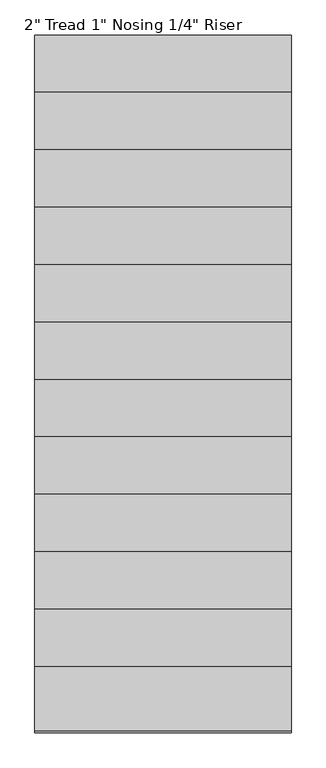
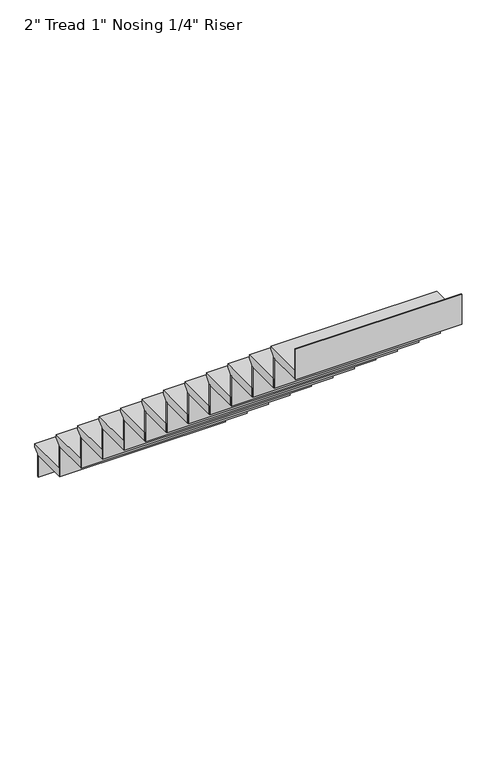
"""IFC4 building model written with IfcOpenShell, lengths in millimetres: stair flight geometry."""

from ifc_helpers import new_model, si_unit, frame, origin, place, context, project, spatial, polyline, outline, extrude, source, transform, mapped, element, save


def stair_flight_7df519db(model_context):
    return source(origin(), model_context, "Body", "SweptSolid", [
        extrude(outline(polyline([(-5623.7944564, -2092.5692308), (-5395.1944564, -2092.5692308), (-5395.1944564, -2111.6192308), (-5420.5944564, -2137.0192308), (-5420.5944564, -2143.3692308), (-5623.7944564, -2143.3692308), (-5623.7944564, -2092.5692308)])), frame((-2404.0095256, 0.0, 0.0), z_axis=(1.0, 0.0, 0.0), x_axis=(0.0, 1.0, 0.0)), (0.0, 0.0, 1.0), 908.05),
        extrude(outline(polyline([(-2404.0095256, -5426.9444564), (-2404.0095256, -5420.5944564), (-1495.9595256, -5420.5944564), (-1495.9595256, -5426.9444564), (-2404.0095256, -5426.9444564)])), frame((0.0, 0.0, -2266.95), z_axis=(0.0, 0.0, 1.0), x_axis=(1.0, 0.0, 0.0)), (0.0, 0.0, 1.0), 123.5807692),
        extrude(outline(polyline([(-2404.0095256, -5630.1444564), (-2404.0095256, -5623.7944564), (-1495.9595256, -5623.7944564), (-1495.9595256, -5630.1444564), (-2404.0095256, -5630.1444564)])), frame((0.0, 0.0, -2143.3692308), z_axis=(0.0, 0.0, 1.0), x_axis=(1.0, 0.0, 0.0)), (0.0, 0.0, 1.0), 174.3807692),
        extrude(outline(polyline([(-5826.9944564, -1918.1884615), (-5598.3944564, -1918.1884615), (-5598.3944564, -1937.2384615), (-5623.7944564, -1962.6384615), (-5623.7944564, -1968.9884615), (-5826.9944564, -1968.9884615), (-5826.9944564, -1918.1884615)])), frame((-2404.0095256, 0.0, 0.0), z_axis=(1.0, 0.0, 0.0), x_axis=(0.0, 1.0, 0.0)), (0.0, 0.0, 1.0), 908.05),
        extrude(outline(polyline([(-2404.0095256, -5833.3444564), (-2404.0095256, -5826.9944564), (-1495.9595256, -5826.9944564), (-1495.9595256, -5833.3444564), (-2404.0095256, -5833.3444564)])), frame((0.0, 0.0, -1968.9884615), z_axis=(0.0, 0.0, 1.0), x_axis=(1.0, 0.0, 0.0)), (0.0, 0.0, 1.0), 174.3807692),
        extrude(outline(polyline([(-6030.1944564, -1743.8076923), (-5801.5944564, -1743.8076923), (-5801.5944564, -1762.8576923), (-5826.9944564, -1788.2576923), (-5826.9944564, -1794.6076923), (-6030.1944564, -1794.6076923), (-6030.1944564, -1743.8076923)])), frame((-2404.0095256, 0.0, 0.0), z_axis=(1.0, 0.0, 0.0), x_axis=(0.0, 1.0, 0.0)), (0.0, 0.0, 1.0), 908.05),
        extrude(outline(polyline([(-2404.0095256, -6036.5444564), (-2404.0095256, -6030.1944564), (-1495.9595256, -6030.1944564), (-1495.9595256, -6036.5444564), (-2404.0095256, -6036.5444564)])), frame((0.0, 0.0, -1794.6076923), z_axis=(0.0, 0.0, 1.0), x_axis=(1.0, 0.0, 0.0)), (0.0, 0.0, 1.0), 174.3807692),
        extrude(outline(polyline([(-6233.3944564, -1569.4269231), (-6004.7944564, -1569.4269231), (-6004.7944564, -1588.4769231), (-6030.1944564, -1613.8769231), (-6030.1944564, -1620.2269231), (-6233.3944564, -1620.2269231), (-6233.3944564, -1569.4269231)])), frame((-2404.0095256, 0.0, 0.0), z_axis=(1.0, 0.0, 0.0), x_axis=(0.0, 1.0, 0.0)), (0.0, 0.0, 1.0), 908.05),
        extrude(outline(polyline([(-2404.0095256, -6239.7444564), (-2404.0095256, -6233.3944564), (-1495.9595256, -6233.3944564), (-1495.9595256, -6239.7444564), (-2404.0095256, -6239.7444564)])), frame((0.0, 0.0, -1620.2269231), z_axis=(0.0, 0.0, 1.0), x_axis=(1.0, 0.0, 0.0)), (0.0, 0.0, 1.0), 174.3807692),
        extrude(outline(polyline([(-6436.5944564, -1395.0461538), (-6207.9944564, -1395.0461538), (-6207.9944564, -1414.0961538), (-6233.3944564, -1439.4961538), (-6233.3944564, -1445.8461538), (-6436.5944564, -1445.8461538), (-6436.5944564, -1395.0461538)])), frame((-2404.0095256, 0.0, 0.0), z_axis=(1.0, 0.0, 0.0), x_axis=(0.0, 1.0, 0.0)), (0.0, 0.0, 1.0), 908.05),
        extrude(outline(polyline([(-2404.0095256, -6442.9444564), (-2404.0095256, -6436.5944564), (-1495.9595256, -6436.5944564), (-1495.9595256, -6442.9444564), (-2404.0095256, -6442.9444564)])), frame((0.0, 0.0, -1445.8461538), z_axis=(0.0, 0.0, 1.0), x_axis=(1.0, 0.0, 0.0)), (0.0, 0.0, 1.0), 174.3807692),
        extrude(outline(polyline([(-6639.7944564, -1220.6653846), (-6411.1944564, -1220.6653846), (-6411.1944564, -1239.7153846), (-6436.5944564, -1265.1153846), (-6436.5944564, -1271.4653846), (-6639.7944564, -1271.4653846), (-6639.7944564, -1220.6653846)])), frame((-2404.0095256, 0.0, 0.0), z_axis=(1.0, 0.0, 0.0), x_axis=(0.0, 1.0, 0.0)), (0.0, 0.0, 1.0), 908.05),
        extrude(outline(polyline([(-2404.0095256, -6646.1444564), (-2404.0095256, -6639.7944564), (-1495.9595256, -6639.7944564), (-1495.9595256, -6646.1444564), (-2404.0095256, -6646.1444564)])), frame((0.0, 0.0, -1271.4653846), z_axis=(0.0, 0.0, 1.0), x_axis=(1.0, 0.0, 0.0)), (0.0, 0.0, 1.0), 174.3807692),
        extrude(outline(polyline([(-6842.9944564, -1046.2846154), (-6614.3944564, -1046.2846154), (-6614.3944564, -1065.3346154), (-6639.7944564, -1090.7346154), (-6639.7944564, -1097.0846154), (-6842.9944564, -1097.0846154), (-6842.9944564, -1046.2846154)])), frame((-2404.0095256, 0.0, 0.0), z_axis=(1.0, 0.0, 0.0), x_axis=(0.0, 1.0, 0.0)), (0.0, 0.0, 1.0), 908.05),
        extrude(outline(polyline([(-2404.0095256, -6849.3444564), (-2404.0095256, -6842.9944564), (-1495.9595256, -6842.9944564), (-1495.9595256, -6849.3444564), (-2404.0095256, -6849.3444564)])), frame((0.0, 0.0, -1097.0846154), z_axis=(0.0, 0.0, 1.0), x_axis=(1.0, 0.0, 0.0)), (0.0, 0.0, 1.0), 174.3807692),
        extrude(outline(polyline([(-7046.1944564, -871.9038462), (-6817.5944564, -871.9038462), (-6817.5944564, -890.9538462), (-6842.9944564, -916.3538462), (-6842.9944564, -922.7038462), (-7046.1944564, -922.7038462), (-7046.1944564, -871.9038462)])), frame((-2404.0095256, 0.0, 0.0), z_axis=(1.0, 0.0, 0.0), x_axis=(0.0, 1.0, 0.0)), (0.0, 0.0, 1.0), 908.05),
        extrude(outline(polyline([(-2404.0095256, -7052.5444564), (-2404.0095256, -7046.1944564), (-1495.9595256, -7046.1944564), (-1495.9595256, -7052.5444564), (-2404.0095256, -7052.5444564)])), frame((0.0, 0.0, -922.7038462), z_axis=(0.0, 0.0, 1.0), x_axis=(1.0, 0.0, 0.0)), (0.0, 0.0, 1.0), 174.3807692),
        extrude(outline(polyline([(-7249.3944564, -697.5230769), (-7020.7944564, -697.5230769), (-7020.7944564, -716.5730769), (-7046.1944564, -741.9730769), (-7046.1944564, -748.3230769), (-7249.3944564, -748.3230769), (-7249.3944564, -697.5230769)])), frame((-2404.0095256, 0.0, 0.0), z_axis=(1.0, 0.0, 0.0), x_axis=(0.0, 1.0, 0.0)), (0.0, 0.0, 1.0), 908.05),
        extrude(outline(polyline([(-2404.0095256, -7255.7444564), (-2404.0095256, -7249.3944564), (-1495.9595256, -7249.3944564), (-1495.9595256, -7255.7444564), (-2404.0095256, -7255.7444564)])), frame((0.0, 0.0, -748.3230769), z_axis=(0.0, 0.0, 1.0), x_axis=(1.0, 0.0, 0.0)), (0.0, 0.0, 1.0), 174.3807692),
        extrude(outline(polyline([(-7452.5944564, -523.1423077), (-7223.9944564, -523.1423077), (-7223.9944564, -542.1923077), (-7249.3944564, -567.5923077), (-7249.3944564, -573.9423077), (-7452.5944564, -573.9423077), (-7452.5944564, -523.1423077)])), frame((-2404.0095256, 0.0, 0.0), z_axis=(1.0, 0.0, 0.0), x_axis=(0.0, 1.0, 0.0)), (0.0, 0.0, 1.0), 908.05),
        extrude(outline(polyline([(-2404.0095256, -7458.9444564), (-2404.0095256, -7452.5944564), (-1495.9595256, -7452.5944564), (-1495.9595256, -7458.9444564), (-2404.0095256, -7458.9444564)])), frame((0.0, 0.0, -573.9423077), z_axis=(0.0, 0.0, 1.0), x_axis=(1.0, 0.0, 0.0)), (0.0, 0.0, 1.0), 174.3807692),
        extrude(outline(polyline([(-7655.7944564, -348.7615385), (-7427.1944564, -348.7615385), (-7427.1944564, -367.8115385), (-7452.5944564, -393.2115385), (-7452.5944564, -399.5615385), (-7655.7944564, -399.5615385), (-7655.7944564, -348.7615385)])), frame((-2404.0095256, 0.0, 0.0), z_axis=(1.0, 0.0, 0.0), x_axis=(0.0, 1.0, 0.0)), (0.0, 0.0, 1.0), 908.05),
        extrude(outline(polyline([(-2404.0095256, -7662.1444564), (-2404.0095256, -7655.7944564), (-1495.9595256, -7655.7944564), (-1495.9595256, -7662.1444564), (-2404.0095256, -7662.1444564)])), frame((0.0, 0.0, -399.5615385), z_axis=(0.0, 0.0, 1.0), x_axis=(1.0, 0.0, 0.0)), (0.0, 0.0, 1.0), 174.3807692),
        extrude(outline(polyline([(-2404.0095256, -7865.3444564), (-2404.0095256, -7858.9944564), (-1495.9595256, -7858.9944564), (-1495.9595256, -7865.3444564), (-2404.0095256, -7865.3444564)])), frame((0.0, 0.0, -225.1807692), z_axis=(0.0, 0.0, 1.0), x_axis=(1.0, 0.0, 0.0)), (0.0, 0.0, 1.0), 174.3807692),
        extrude(outline(polyline([(-7858.9944564, -174.3807692), (-7630.3944564, -174.3807692), (-7630.3944564, -193.4307692), (-7655.7944564, -218.8307692), (-7655.7944564, -225.1807692), (-7858.9944564, -225.1807692), (-7858.9944564, -174.3807692)])), frame((-2404.0095256, 0.0, 0.0), z_axis=(1.0, 0.0, 0.0), x_axis=(0.0, 1.0, 0.0)), (0.0, 0.0, 1.0), 908.05),
    ])


if __name__ == "__main__":
    model = new_model("IFC4")
    model_context = context("Model", 3, world=origin())
    ifc_project = project(units=[si_unit("LENGTHUNIT", "METRE", prefix="MILLI")], contexts=[model_context])
    site = spatial("IfcSite", under=ifc_project)
    building = spatial("IfcBuilding", under=site)
    placement = place(None, origin())
    stair_flight_shape = stair_flight_7df519db(model_context)
    element("IfcStairFlight", 1, ObjectType="2\" Tread 1\" Nosing 1/4\" Riser", at=placement, inside=building, context=model_context, shape_type="MappedRepresentation", body=[
        mapped(stair_flight_shape, transform((0.0, 0.0, 0.0), x_axis=(1.0, 0.0, 0.0), y_axis=(0.0, 1.0, 0.0), z_axis=(0.0, 0.0, 1.0))),
    ])
    save(model, "model.ifc")
